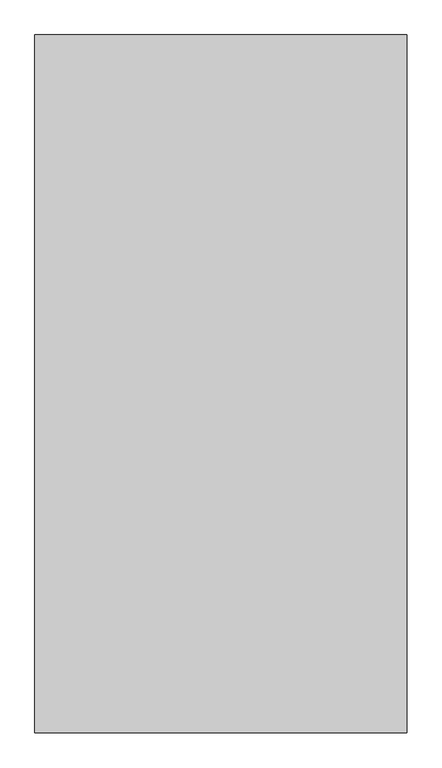
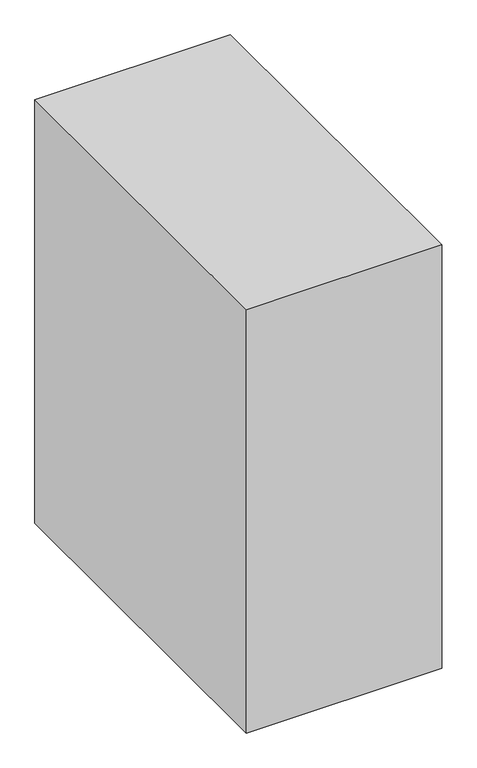
"""IFC4 building model written with IfcOpenShell, lengths in millimetres: proxy geometry, Space Planning Box_hec : Space Planning Box_hec."""

import ifcopenshell
import ifcopenshell.guid

model = None  # the IFC model being written
_history = None  # IfcOwnerHistory: only IFC2X3 demands one
_inside = {}  # id of a spatial element -> (the spatial element, [elements in it])
_under = {}  # id of a project, library or spatial element -> (it, [spatial elements below it])
_declared = {}  # id of a project -> (the project, [libraries it declares])
_typed = {}  # id of a type object -> (the type object, [elements of that type])
_made_of = {}  # id of a material, layer set ... -> (it, [elements and type objects made of it])


def new_model(schema):
    """Start an empty IFC model of exactly this schema.

    Asked for "IFC4X3", IfcOpenShell would pick the latest addendum, in which some entities
    have other attributes; the version numbers below select the first issue.
    IFC2X3 requires an IfcOwnerHistory on every rooted entity: one is made here for all.
    """
    global model, _history
    if schema == "IFC4X3":
        model = ifcopenshell.file(schema_version=(4, 3, 0, 0))
    else:
        model = ifcopenshell.file(schema=schema)
    _inside.clear()
    _under.clear()
    _declared.clear()
    _typed.clear()
    _made_of.clear()
    _history = None
    if model.schema == "IFC2X3":
        org = make("IfcOrganization", Name="unknown")
        user = make(
            "IfcPersonAndOrganization",
            ThePerson=make("IfcPerson", FamilyName="unknown"),
            TheOrganization=org,
        )
        app = make(
            "IfcApplication",
            ApplicationDeveloper=org,
            Version="unknown",
            ApplicationFullName="unknown",
            ApplicationIdentifier="unknown",
        )
        _history = make(
            "IfcOwnerHistory",
            OwningUser=user,
            OwningApplication=app,
            ChangeAction="ADDED",
            CreationDate=0,
        )
    return model


def make(cls, **values):
    """One entity of the class cls with the attributes given. An attribute that is None is left unset."""
    return model.create_entity(
        cls, **{name: value for name, value in values.items() if value is not None}
    )


def rooted(cls, **values):
    """An entity with a GlobalId (a new one), such as an element, a storey or a relation."""
    return make(cls, GlobalId=ifcopenshell.guid.new(), OwnerHistory=_history, **values)


def si_unit(unit_type, name, prefix=None):
    """IfcSIUnit, for example si_unit("LENGTHUNIT", "METRE", prefix="MILLI")."""
    return make("IfcSIUnit", UnitType=unit_type, Prefix=prefix, Name=name)


def assignment(units):
    """IfcUnitAssignment: the units of a project."""
    return None if units is None else make("IfcUnitAssignment", Units=units)


def point(xyz):
    """IfcCartesianPoint."""
    return None if xyz is None else make("IfcCartesianPoint", Coordinates=xyz)


def direction(xyz):
    """IfcDirection."""
    return None if xyz is None else make("IfcDirection", DirectionRatios=xyz)


def frame(location, z_axis=None, x_axis=None):
    """IfcAxis2Placement3D, a coordinate frame: its origin and axes. An axis left out is left unset."""
    return make(
        "IfcAxis2Placement3D",
        Location=point(location),
        Axis=direction(z_axis),
        RefDirection=direction(x_axis),
    )


def origin():
    """The frame at (0, 0, 0) with its axes left unset."""
    return frame((0.0, 0.0, 0.0))


def origin_with_axes():
    """The frame at (0, 0, 0) with the z axis (0, 0, 1) and the x axis (1, 0, 0) written out."""
    return frame((0.0, 0.0, 0.0), z_axis=(0.0, 0.0, 1.0), x_axis=(1.0, 0.0, 0.0))


def place(relative_to, where):
    """IfcLocalPlacement: puts the frame where relative to a parent placement (None: the world)."""
    return make(
        "IfcLocalPlacement", PlacementRelTo=relative_to, RelativePlacement=where
    )


def context(
    kind, dimensions, precision=None, world=None, true_north=None, identifier=None
):
    """IfcGeometricRepresentationContext, for example the 3D "Model" context."""
    return make(
        "IfcGeometricRepresentationContext",
        ContextIdentifier=identifier,
        ContextType=kind,
        CoordinateSpaceDimension=dimensions,
        Precision=precision,
        WorldCoordinateSystem=world,
        TrueNorth=true_north,
    )


def project(units=None, contexts=None):
    """IfcProject with its units and contexts."""
    return rooted(
        "IfcProject",
        Name="project",
        RepresentationContexts=contexts,
        UnitsInContext=assignment(units),
    )


def spatial(cls, under=None, at=None, **own):
    """A site, building, storey or space (cls), placed at a placement, below another one or the project."""
    s = rooted(cls, ObjectPlacement=at, **own)
    if under is not None:
        _under.setdefault(under.id(), (under, []))[1].append(s)
    return s


def polyline(points):
    """IfcPolyline through the points."""
    return make("IfcPolyline", Points=[point(p) for p in points])


def outline(outer, holes=None, kind="AREA"):
    """IfcArbitraryClosedProfileDef: a profile drawn as a closed curve; with holes, ...WithVoids."""
    if holes is None:
        return make("IfcArbitraryClosedProfileDef", ProfileType=kind, OuterCurve=outer)
    return make(
        "IfcArbitraryProfileDefWithVoids",
        ProfileType=kind,
        OuterCurve=outer,
        InnerCurves=holes,
    )


def extrude(swept, where, along, depth):
    """IfcExtrudedAreaSolid: the profile swept, set in the frame where, extruded along a direction by depth."""
    return make(
        "IfcExtrudedAreaSolid",
        SweptArea=swept,
        Position=where,
        ExtrudedDirection=direction(along),
        Depth=depth,
    )


def shape(context_of_items, identifier, shape_type, items):
    """IfcShapeRepresentation: the items that make up one representation, for example the "Body"."""
    return make(
        "IfcShapeRepresentation",
        ContextOfItems=context_of_items,
        RepresentationIdentifier=identifier,
        RepresentationType=shape_type,
        Items=items,
    )


def source(mapping_origin, context_of_items, identifier, shape_type, items):
    """IfcRepresentationMap: a shape defined once, which mapped items show again and again."""
    return make(
        "IfcRepresentationMap",
        MappingOrigin=mapping_origin,
        MappedRepresentation=shape(context_of_items, identifier, shape_type, items),
    )


def transform(
    local_origin,
    x_axis=None,
    y_axis=None,
    z_axis=None,
    scale=None,
    scale2=None,
    scale3=None,
    uniform=True,
):
    """IfcCartesianTransformationOperator3D, or its non-uniform kind. x_axis, y_axis, z_axis: its Axis1, 2, 3."""
    if uniform:
        return make(
            "IfcCartesianTransformationOperator3D",
            Axis1=direction(x_axis),
            Axis2=direction(y_axis),
            LocalOrigin=point(local_origin),
            Scale=scale,
            Axis3=direction(z_axis),
        )
    return make(
        "IfcCartesianTransformationOperator3DnonUniform",
        Axis1=direction(x_axis),
        Axis2=direction(y_axis),
        LocalOrigin=point(local_origin),
        Scale=scale,
        Axis3=direction(z_axis),
        Scale2=scale2,
        Scale3=scale3,
    )


def mapped(mapping_source, mapping_target):
    """IfcMappedItem: shows the shape of a source again, moved by a transform."""
    return make(
        "IfcMappedItem", MappingSource=mapping_source, MappingTarget=mapping_target
    )


def made_of(thing, what):
    """Note that an element or type object is made of a material, layer set ...; save() writes the relation."""
    if what is not None:
        _made_of.setdefault(what.id(), (what, []))[1].append(thing)
    return thing


def element(
    cls,
    number,
    at=None,
    inside=None,
    cuts=None,
    type_object=None,
    material=None,
    context=None,
    identifier="Body",
    shape_type=None,
    held_by="IfcProductDefinitionShape",
    body=None,
    shapes=None,
    **own,
):
    """One element of the class cls, such as IfcWall. Its Tag is "e" and its number.

    at: its placement. inside: the storey or other place that contains it. cuts: it is an
    opening in that element (IfcRelVoidsElement). A single representation is given by context,
    identifier, shape_type and body (its items); several are given by shapes. held_by: the class
    of the entity that holds the representations. save() writes the other relations.
    """
    e = rooted(cls, Tag="e%d" % number, ObjectPlacement=at, **own)
    if body is not None:
        shapes = [shape(context, identifier, shape_type, body)]
    if shapes is not None:
        e.Representation = make(held_by, Representations=shapes)
    if inside is not None:
        _inside.setdefault(inside.id(), (inside, []))[1].append(e)
    if cuts is not None:
        rooted(
            "IfcRelVoidsElement", RelatingBuildingElement=cuts, RelatedOpeningElement=e
        )
    if type_object is not None:
        _typed.setdefault(type_object.id(), (type_object, []))[1].append(e)
    return made_of(e, material)


def aggregate(whole, parts):
    """IfcRelAggregates: a whole, such as a stair, and the parts it consists of."""
    return rooted("IfcRelAggregates", RelatingObject=whole, RelatedObjects=parts)


def save(model, path):
    """Write the relations noted so far, then the file.

    IfcRelAggregates (storeys below a building ...), IfcRelContainedInSpatialStructure (elements
    in a storey), IfcRelDefinesByType, IfcRelAssociatesMaterial and IfcRelDeclares: one each for
    every whole, place, type object, material and project.
    """
    for whole, parts in _under.values():
        aggregate(whole, parts)
    for where, things in _inside.values():
        rooted(
            "IfcRelContainedInSpatialStructure",
            RelatedElements=things,
            RelatingStructure=where,
        )
    for kind, things in _typed.values():
        rooted("IfcRelDefinesByType", RelatedObjects=things, RelatingType=kind)
    for what, things in _made_of.values():
        rooted("IfcRelAssociatesMaterial", RelatedObjects=things, RelatingMaterial=what)
    for by, libraries in _declared.values():
        rooted("IfcRelDeclares", RelatingContext=by, RelatedDefinitions=libraries)
    model.write(path)


def generic_models_570012e4(model_context):
    return source(origin(), model_context, "Body", "SweptSolid", [
        extrude(outline(polyline([(1200.0, 2250.0), (1200.0, -2250.0), (-1200.0, -2250.0), (-1200.0, 2250.0), (1200.0, 2250.0)])), origin_with_axes(), (0.0, 0.0, 1.0), 5500.0),
    ])


if __name__ == "__main__":
    model = new_model("IFC4")
    model_context = context("Model", 3, world=origin())
    ifc_project = project(units=[si_unit("LENGTHUNIT", "METRE", prefix="MILLI")], contexts=[model_context])
    site = spatial("IfcSite", under=ifc_project)
    building = spatial("IfcBuilding", under=site)
    placement = place(None, origin())
    generic_models_shape = generic_models_570012e4(model_context)
    element("IfcBuildingElementProxy", 1, Name="Space Planning Box_hec : Space Planning Box_hec", ObjectType="Space Planning Box_hec : Space Planning Box_hec", at=placement, inside=building, context=model_context, shape_type="MappedRepresentation", body=[
        mapped(generic_models_shape, transform((0.0, 0.0, 0.0), x_axis=(1.0, 0.0, 0.0), y_axis=(0.0, 1.0, 0.0), z_axis=(0.0, 0.0, 1.0))),
    ])
    save(model, "model.ifc")

# Revit data of these elements
# Type "Space Planning Box_hec : Space Planning Box_hec"
#   Type Comments = "..."
#   Room Name [instance default] = "?"
#   Interior Finish [instance default] = ""
#   Exterior Finish [instance default] = ""
#   Department [instance default] = ""
#   Assembly Code = "..."
#   Width [instance default] = 1524 mm
#   Program Area [instance default] = 0.00 m²
#   Length [instance default] = 1524 mm
#   Height [instance default] = 1524 mm
#   Area [instance default] = 2.32258 m²
#   Fill Color [instance default] = Cyan
#   Default Elevation = 0
# Element 1 (IfcBuildingElementProxy, "Space Planning Box_hec : Space Planning Box_hec")
#   Room Name = "Duct Shaft"
#   Department = "PATHV3"
#   Width = 2400 mm
#   Program Area = 10.80 m²
#   Length = 4500 mm
#   Height = 5500 mm
#   Area = 10.80 m²
#   Fill Color = Lavender
#   Materials on its faces: "Lavender"
# Materials
#   "Cyan": class "Generic", colour RGB 0 255 255, transparency 0.2, Cost = 0
#   "Lavender": class "Generic", colour RGB 186 85 211, transparency 0.2, Cost = 0
